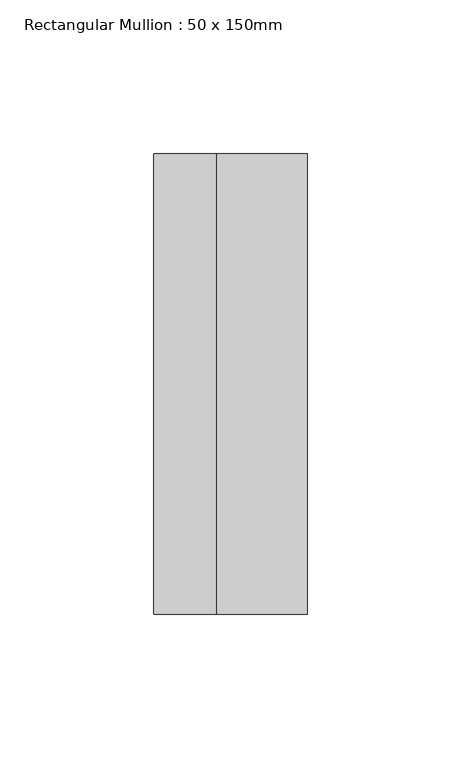
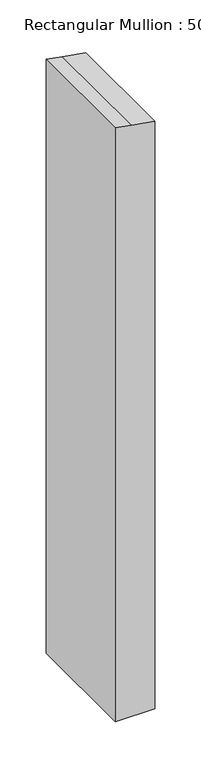
"""IFC4 building model written with IfcOpenShell, lengths in millimetres: member geometry, Rectangular Mullion : 50 x 150mm."""

from ifc_helpers import new_model, si_unit, frame, origin, place, context, project, spatial, polyline, outline, extrude, source, transform, mapped, element, save


def rectangular_mullion_50_x_150mm_6a3808df(model_context):
    return source(origin(), model_context, "Body", "SweptSolid", [
        extrude(outline(polyline([(-4.7938398, 25.0), (0.3798062, -4.3412044), (4.0225092, -25.0), (-783.9384156, -25.0), (-783.9384156, 25.0), (-4.7938398, 25.0)])), frame((0.0, -75.0, 0.0), z_axis=(0.0, 1.0, 0.0), x_axis=(0.0, 0.0, 1.0)), (0.0, 0.0, 1.0), 150.0),
    ])


if __name__ == "__main__":
    model = new_model("IFC4")
    model_context = context("Model", 3, world=origin())
    ifc_project = project(units=[si_unit("LENGTHUNIT", "METRE", prefix="MILLI")], contexts=[model_context])
    site = spatial("IfcSite", under=ifc_project)
    building = spatial("IfcBuilding", under=site)
    placement = place(None, origin())
    rectangular_mullion_50_x_150mm_shape = rectangular_mullion_50_x_150mm_6a3808df(model_context)
    element("IfcMember", 1, ObjectType="Rectangular Mullion : 50 x 150mm", at=placement, inside=building, context=model_context, shape_type="MappedRepresentation", body=[
        mapped(rectangular_mullion_50_x_150mm_shape, transform((0.0, 0.0, 0.0), x_axis=(1.0, 0.0, 0.0), y_axis=(0.0, 1.0, 0.0), z_axis=(0.0, 0.0, 1.0))),
    ])
    save(model, "model.ifc")

# Revit data of these elements
# Project information
#   Project Issue Date = "Issue Date"
#   Project Status = "Project Status"
#   Client Name = "Owner"
#   Project Address = "Enter address here"
#   Project Name = "Project Name"
#   Project Number = "0001"
# Type "Rectangular Mullion : 50 x 150mm"
#   built-in parameter 1007304 = 0.492126 (stored number, unit not read)
#   built-in parameter 1007301 = 0.082021 (stored number, unit not read)
#   built-in parameter 1007300 = 0.082021 (stored number, unit not read)
# Element 1 (IfcMember, "Rectangular Mullion : 50 x 150mm")
#   Materials on its faces: "Aluminium"
# Materials
#   "Aluminium": class "Metal", colour RGB 247 247 247, transparency 0, Description = "Aluminium 6061", Cost = 0
